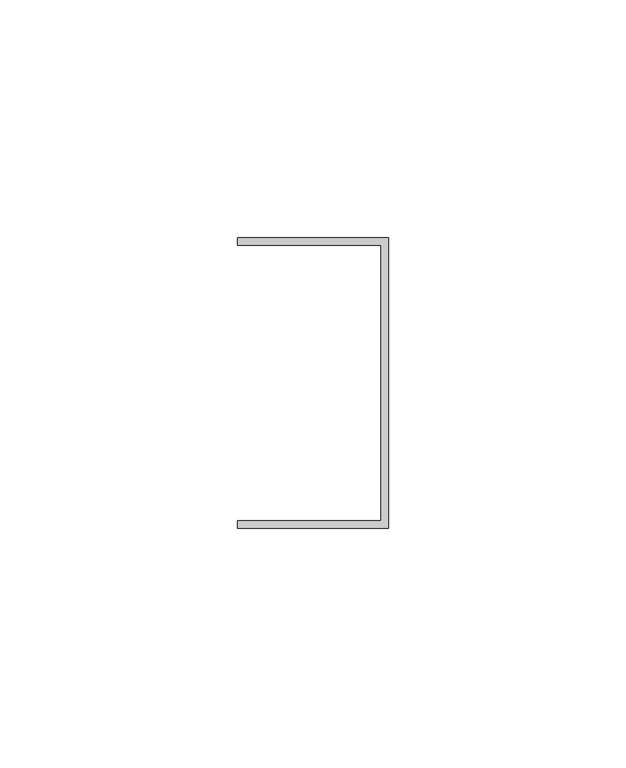
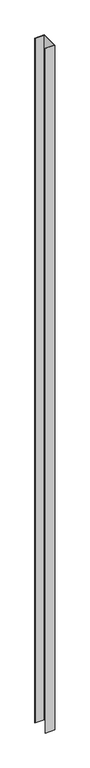
"""IFC4 building model written with IfcOpenShell, lengths in millimetres: proxy geometry, Generic Models 7:Generic Models 1:3:Generic Models 1:3 : Generic Models 7:Generic Models 1:305549:3:Generic Models 1:3:Generic Models 1:3 : Generic Models 7:Generic Models 1:305549:3 : Generic Models 7:Generic Models 1:3:Generic Models 1:3 : Generic Models 7:Generic Models 1:305549:301244:35 : Generic Models 7:Generic Models 1:3:Generic Models 1:3 : Generic Models 7:Generic Models 1:305549:3:Generic Models 1:3:Generic Models 1:3 : Generic Models 7:Generic Models 1:305549:3 : Generic Models 7:Generic Models 1:3:Generic Models 1:3 : Generic Models 7:Generic Models 1:305549:301244:308848."""

from ifc_helpers import new_model, si_unit, frame, origin, place, context, project, spatial, polyline, outline, extrude, source, transform, mapped, element, save


def generic_models_1663d69c(model_context):
    return source(origin(), model_context, "Body", "SweptSolid", [
        extrude(outline(polyline([(596163.786724, -579015.772634), (596163.786724, -579076.8913841), (596132.036724, -579076.8913841), (596132.036724, -579075.3038841), (596162.199224, -579075.3038841), (596162.199224, -579017.360134), (596132.036724, -579017.360134), (596132.036724, -579015.772634), (596163.786724, -579015.772634)])), frame((0.0, 0.0, 50.8), z_axis=(0.0, 0.0, 1.0), x_axis=(1.0, 0.0, 0.0)), (0.0, 0.0, 1.0), 2430.9324376),
    ])


if __name__ == "__main__":
    model = new_model("IFC4")
    model_context = context("Model", 3, world=origin())
    ifc_project = project(units=[si_unit("LENGTHUNIT", "METRE", prefix="MILLI")], contexts=[model_context])
    site = spatial("IfcSite", under=ifc_project)
    building = spatial("IfcBuilding", under=site)
    placement = place(None, origin())
    generic_models_shape = generic_models_1663d69c(model_context)
    element("IfcBuildingElementProxy", 1, Name="Generic Models 7:Generic Models 1:3:Generic Models 1:3 : Generic Models 7:Generic Models 1:305549:3:Generic Models 1:3:Generic Models 1:3 : Generic Models 7:Generic Models 1:305549:3 : Generic Models 7:Generic Models 1:3:Generic Models 1:3 : Generic Models 7:Generic Models 1:305549:301244:35 : Generic Models 7:Generic Models 1:3:Generic Models 1:3 : Generic Models 7:Generic Models 1:305549:3:Generic Models 1:3:Generic Models 1:3 : Generic Models 7:Generic Models 1:305549:3 : Generic Models 7:Generic Models 1:3:Generic Models 1:3 : Generic Models 7:Generic Models 1:305549:301244:308848", ObjectType="Generic Models 7:Generic Models 1:3:Generic Models 1:3 : Generic Models 7:Generic Models 1:305549:3:Generic Models 1:3:Generic Models 1:3 : Generic Models 7:Generic Models 1:305549:3 : Generic Models 7:Generic Models 1:3:Generic Models 1:3 : Generic Models 7:Generic Models 1:305549:301244:35 : Generic Models 7:Generic Models 1:3:Generic Models 1:3 : Generic Models 7:Generic Models 1:305549:3:Generic Models 1:3:Generic Models 1:3 : Generic Models 7:Generic Models 1:305549:3 : Generic Models 7:Generic Models 1:3:Generic Models 1:3 : Generic Models 7:Generic Models 1:305549:301244:308848", at=placement, inside=building, context=model_context, shape_type="MappedRepresentation", body=[
        mapped(generic_models_shape, transform((0.0, 0.0, 0.0), x_axis=(1.0, 0.0, 0.0), y_axis=(0.0, 1.0, 0.0), z_axis=(0.0, 0.0, 1.0))),
    ])
    save(model, "model.ifc")

# Revit data of these elements
# Type "Generic Models 7:Generic Models 1:3:Generic Models 1:3 : Generic Models 7:Generic Models 1:305549:3:Generic Models 1:3:Generic Models 1:3 : Generic Models 7:Generic Models 1:305549:3 : Generic Models 7:Generic Models 1:3:Generic Models 1:3 : Generic Models 7:Generic Models 1:305549:301244:35 : Generic Models 7:Generic Models 1:3:Generic Models 1:3 : Generic Models 7:Generic Models 1:305549:3:Generic Models 1:3:Generic Models 1:3 : Generic Models 7:Generic Models 1:305549:3 : Generic Models 7:Generic Models 1:3:Generic Models 1:3 : Generic Models 7:Generic Models 1:305549:301244:308848"
#   NameOverride = "Generic Models 7:Generic Models 1:3:Generic Models 1:3 : Generic Models 7:Generic Models 1:305549:3:Generic Models 1:3:Generic Models 1:3 : Generic Models 7:Generic Models 1:305549:3 : Generic Models 7:Generic Models 1:3:Generic Models 1:3 : Generic Models 7:Generic Models 1:305549:301244:308848"
#   ObjectTypeOverride = "Generic Models 1:3:Generic Models 1:3 : Generic Models 7:Generic Models 1:305549:3 : Generic Models 7:Generic Models 1:3:Generic Models 1:3 : Generic Models 7:Generic Models 1:305549:301244"
#   Reference = "Generic Models 1"
#   Tag = "308848"
# Element 1 (IfcBuildingElementProxy, "Generic Models 7:Generic Models 1:3:Generic Models 1:3 : Generic Models 7:Generic Models 1:305549:3:Generic Models 1:3:Generic Models 1:3 : Generic Models 7:Generic Models 1:305549:3 : Generic Models 7:Generic Models 1:3:Generic Models 1:3 : Generic Models 7:Generic Models 1:305549:301244:35 : Generic Models 7:Generic Models 1:3:Generic Models 1:3 : Generic Models 7:Generic Models 1:305549:3:Generic Models 1:3:Generic Models 1:3 : Generic Models 7:Generic Models 1:305549:3 : Generic Models 7:Generic Models 1:3:Generic Models 1:3 : Generic Models 7:Generic Models 1:305549:301244:308848")
#   Materials on its faces: "GALVANIZED U-CHANNEL (250T125-33)"
# Materials
#   "GALVANIZED U-CHANNEL (250T125-33)": class "Unassigned", colour RGB 202 201 200, transparency 0, Keynote = "M05451300.02", Cost = 0
